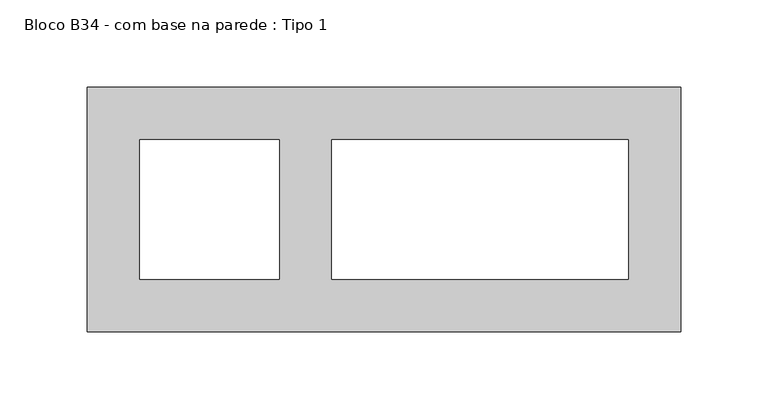
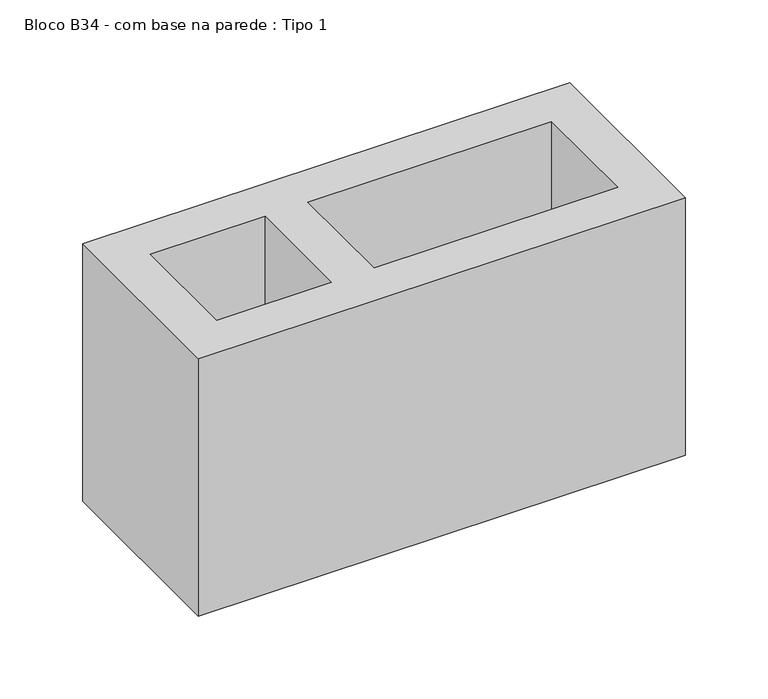
"""IFC4 building model written with IfcOpenShell, lengths in millimetres: proxy geometry, Bloco B34 - com base na parede : Tipo 1."""

from ifc_helpers import new_model, si_unit, origin, origin_with_axes, place, context, project, spatial, polyline, outline, extrude, source, transform, mapped, element, save


def bloco_b34_com_base_na_parede_tipo_1_a1f5d4d2(model_context):
    return source(origin(), model_context, "Body", "SweptSolid", [
        extrude(outline(polyline([(295.0, 70.0), (295.0, -70.0), (-45.0, -70.0), (-45.0, 70.0), (295.0, 70.0)]), holes=[polyline([(65.0, 40.0), (-15.0, 40.0), (-15.0, -40.0), (65.0, -40.0), (65.0, 40.0)]), polyline([(95.0, 40.0), (95.0, -40.0), (265.0, -40.0), (265.0, 40.0), (95.0, 40.0)])]), origin_with_axes(), (0.0, 0.0, 1.0), 190.0),
    ])


if __name__ == "__main__":
    model = new_model("IFC4")
    model_context = context("Model", 3, world=origin())
    ifc_project = project(units=[si_unit("LENGTHUNIT", "METRE", prefix="MILLI")], contexts=[model_context])
    site = spatial("IfcSite", under=ifc_project)
    building = spatial("IfcBuilding", under=site)
    placement = place(None, origin())
    bloco_b34_com_base_na_parede_tipo_1_shape = bloco_b34_com_base_na_parede_tipo_1_a1f5d4d2(model_context)
    element("IfcBuildingElementProxy", 1, Name="Bloco B34 - com base na parede : Tipo 1", ObjectType="Bloco B34 - com base na parede : Tipo 1", at=placement, inside=building, context=model_context, shape_type="MappedRepresentation", body=[
        mapped(bloco_b34_com_base_na_parede_tipo_1_shape, transform((0.0, 0.0, 0.0), x_axis=(1.0, 0.0, 0.0), y_axis=(0.0, 1.0, 0.0), z_axis=(0.0, 0.0, 1.0))),
    ])
    save(model, "model.ifc")

# Revit data of these elements
# Type "Bloco B34 - com base na parede : Tipo 1"
#   SINAPI = ""
#   Assembly Code = ""
